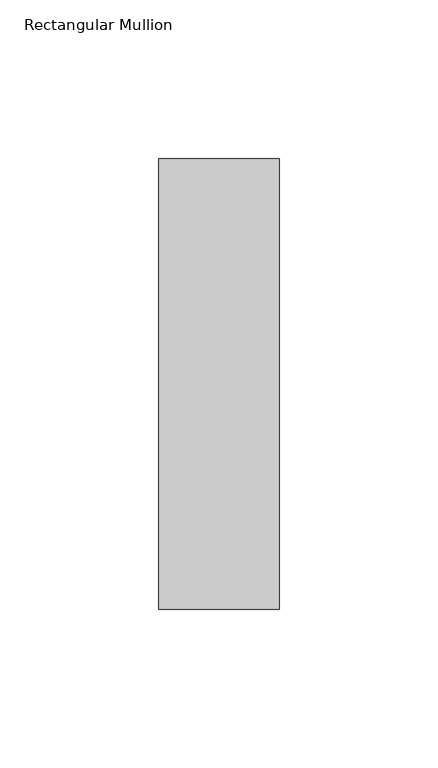
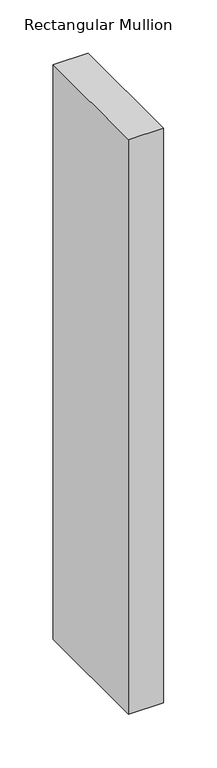
"""IFC4 building model written with IfcOpenShell, lengths in millimetres: member geometry, Rectangular Mullion : NLRS_21_CWM_hsb-regel 38x142_gen_rsf."""

from ifc_helpers import new_model, si_unit, frame, origin, place, context, project, spatial, polyline, outline, extrude, source, transform, mapped, element, save


def rectangular_mullion_0fff75b4(model_context):
    return source(origin(), model_context, "Body", "SweptSolid", [
        extrude(outline(polyline([(19.0, -71.0), (-19.0, -71.0), (-19.0, 71.0), (19.0, 71.0), (19.0, -71.0)])), frame((0.0, 0.0, -659.0), z_axis=(0.0, 0.0, 1.0), x_axis=(1.0, 0.0, 0.0)), (0.0, 0.0, 1.0), 659.0),
    ])


if __name__ == "__main__":
    model = new_model("IFC4")
    model_context = context("Model", 3, world=origin())
    ifc_project = project(units=[si_unit("LENGTHUNIT", "METRE", prefix="MILLI")], contexts=[model_context])
    site = spatial("IfcSite", under=ifc_project)
    building = spatial("IfcBuilding", under=site)
    placement = place(None, origin())
    rectangular_mullion_shape = rectangular_mullion_0fff75b4(model_context)
    element("IfcMember", 1, ObjectType="Rectangular Mullion : NLRS_21_CWM_hsb-regel 38x142_gen_rsf", at=placement, inside=building, context=model_context, shape_type="MappedRepresentation", body=[
        mapped(rectangular_mullion_shape, transform((0.0, 0.0, 0.0), x_axis=(1.0, 0.0, 0.0), y_axis=(0.0, 1.0, 0.0), z_axis=(0.0, 0.0, 1.0))),
    ])
    save(model, "model.ifc")

# Revit data of these elements
# Type "Rectangular Mullion : NLRS_21_CWM_hsb-regel 38x142_gen_rsf"
#   Export Type to IFC As = "IfcWall"
#   Type IfcGUID = "07M7mRoiH1CR8m_RSKIwpF"
#   Assembly Code = "21.10"
#   built-in parameter 1007322 = 0.465879 (stored number, unit not read)
#   built-in parameter 1007321 = 0.062336 (stored number, unit not read)
#   built-in parameter 1007320 = 0.062336 (stored number, unit not read)
# Element 1 (IfcMember, "Rectangular Mullion : NLRS_21_CWM_hsb-regel 38x142_gen_rsf")
#   Materials on its faces: "NLRS_i2_hout naaldhout vuren_gen_rsf"
# Materials
#   "NLRS_i2_hout naaldhout vuren_gen_rsf": class "I - Hout", colour RGB 234 199 147, transparency 0, Keynote = "i2", Manufacturer = "Revit Standards Foundation", URL = "www.revitstandards.org", Description = "hout vuren", Cost = 0
